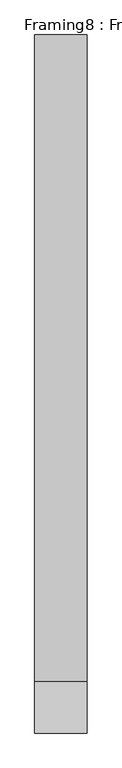
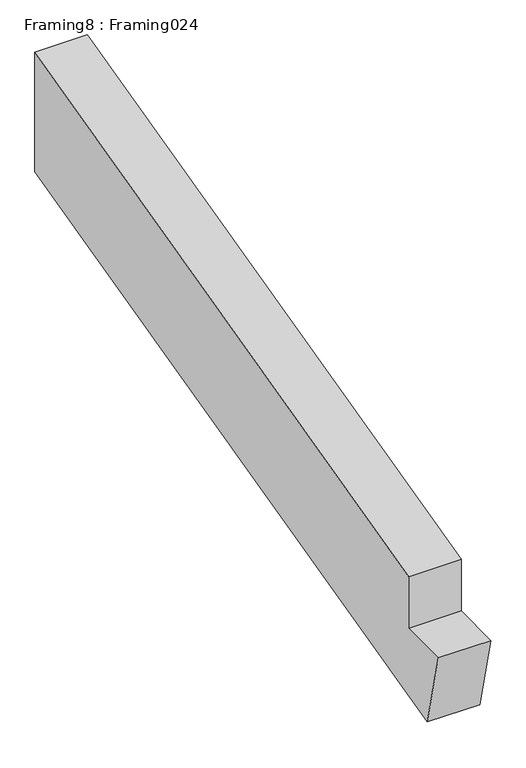
"""IFC4 building model written with IfcOpenShell, lengths in millimetres: proxy geometry, Framing8 : Framing024."""

import ifcopenshell
import ifcopenshell.guid

model = None  # the IFC model being written
_history = None  # IfcOwnerHistory: only IFC2X3 demands one
_inside = {}  # id of a spatial element -> (the spatial element, [elements in it])
_under = {}  # id of a project, library or spatial element -> (it, [spatial elements below it])
_declared = {}  # id of a project -> (the project, [libraries it declares])
_typed = {}  # id of a type object -> (the type object, [elements of that type])
_made_of = {}  # id of a material, layer set ... -> (it, [elements and type objects made of it])


def new_model(schema):
    """Start an empty IFC model of exactly this schema.

    Asked for "IFC4X3", IfcOpenShell would pick the latest addendum, in which some entities
    have other attributes; the version numbers below select the first issue.
    IFC2X3 requires an IfcOwnerHistory on every rooted entity: one is made here for all.
    """
    global model, _history
    if schema == "IFC4X3":
        model = ifcopenshell.file(schema_version=(4, 3, 0, 0))
    else:
        model = ifcopenshell.file(schema=schema)
    _inside.clear()
    _under.clear()
    _declared.clear()
    _typed.clear()
    _made_of.clear()
    _history = None
    if model.schema == "IFC2X3":
        org = make("IfcOrganization", Name="unknown")
        user = make(
            "IfcPersonAndOrganization",
            ThePerson=make("IfcPerson", FamilyName="unknown"),
            TheOrganization=org,
        )
        app = make(
            "IfcApplication",
            ApplicationDeveloper=org,
            Version="unknown",
            ApplicationFullName="unknown",
            ApplicationIdentifier="unknown",
        )
        _history = make(
            "IfcOwnerHistory",
            OwningUser=user,
            OwningApplication=app,
            ChangeAction="ADDED",
            CreationDate=0,
        )
    return model


def make(cls, **values):
    """One entity of the class cls with the attributes given. An attribute that is None is left unset."""
    return model.create_entity(
        cls, **{name: value for name, value in values.items() if value is not None}
    )


def rooted(cls, **values):
    """An entity with a GlobalId (a new one), such as an element, a storey or a relation."""
    return make(cls, GlobalId=ifcopenshell.guid.new(), OwnerHistory=_history, **values)


def si_unit(unit_type, name, prefix=None):
    """IfcSIUnit, for example si_unit("LENGTHUNIT", "METRE", prefix="MILLI")."""
    return make("IfcSIUnit", UnitType=unit_type, Prefix=prefix, Name=name)


def assignment(units):
    """IfcUnitAssignment: the units of a project."""
    return None if units is None else make("IfcUnitAssignment", Units=units)


def point(xyz):
    """IfcCartesianPoint."""
    return None if xyz is None else make("IfcCartesianPoint", Coordinates=xyz)


def direction(xyz):
    """IfcDirection."""
    return None if xyz is None else make("IfcDirection", DirectionRatios=xyz)


def frame(location, z_axis=None, x_axis=None):
    """IfcAxis2Placement3D, a coordinate frame: its origin and axes. An axis left out is left unset."""
    return make(
        "IfcAxis2Placement3D",
        Location=point(location),
        Axis=direction(z_axis),
        RefDirection=direction(x_axis),
    )


def origin():
    """The frame at (0, 0, 0) with its axes left unset."""
    return frame((0.0, 0.0, 0.0))


def place(relative_to, where):
    """IfcLocalPlacement: puts the frame where relative to a parent placement (None: the world)."""
    return make(
        "IfcLocalPlacement", PlacementRelTo=relative_to, RelativePlacement=where
    )


def context(
    kind, dimensions, precision=None, world=None, true_north=None, identifier=None
):
    """IfcGeometricRepresentationContext, for example the 3D "Model" context."""
    return make(
        "IfcGeometricRepresentationContext",
        ContextIdentifier=identifier,
        ContextType=kind,
        CoordinateSpaceDimension=dimensions,
        Precision=precision,
        WorldCoordinateSystem=world,
        TrueNorth=true_north,
    )


def project(units=None, contexts=None):
    """IfcProject with its units and contexts."""
    return rooted(
        "IfcProject",
        Name="project",
        RepresentationContexts=contexts,
        UnitsInContext=assignment(units),
    )


def spatial(cls, under=None, at=None, **own):
    """A site, building, storey or space (cls), placed at a placement, below another one or the project."""
    s = rooted(cls, ObjectPlacement=at, **own)
    if under is not None:
        _under.setdefault(under.id(), (under, []))[1].append(s)
    return s


def polyline(points):
    """IfcPolyline through the points."""
    return make("IfcPolyline", Points=[point(p) for p in points])


def outline(outer, holes=None, kind="AREA"):
    """IfcArbitraryClosedProfileDef: a profile drawn as a closed curve; with holes, ...WithVoids."""
    if holes is None:
        return make("IfcArbitraryClosedProfileDef", ProfileType=kind, OuterCurve=outer)
    return make(
        "IfcArbitraryProfileDefWithVoids",
        ProfileType=kind,
        OuterCurve=outer,
        InnerCurves=holes,
    )


def extrude(swept, where, along, depth):
    """IfcExtrudedAreaSolid: the profile swept, set in the frame where, extruded along a direction by depth."""
    return make(
        "IfcExtrudedAreaSolid",
        SweptArea=swept,
        Position=where,
        ExtrudedDirection=direction(along),
        Depth=depth,
    )


def shape(context_of_items, identifier, shape_type, items):
    """IfcShapeRepresentation: the items that make up one representation, for example the "Body"."""
    return make(
        "IfcShapeRepresentation",
        ContextOfItems=context_of_items,
        RepresentationIdentifier=identifier,
        RepresentationType=shape_type,
        Items=items,
    )


def source(mapping_origin, context_of_items, identifier, shape_type, items):
    """IfcRepresentationMap: a shape defined once, which mapped items show again and again."""
    return make(
        "IfcRepresentationMap",
        MappingOrigin=mapping_origin,
        MappedRepresentation=shape(context_of_items, identifier, shape_type, items),
    )


def transform(
    local_origin,
    x_axis=None,
    y_axis=None,
    z_axis=None,
    scale=None,
    scale2=None,
    scale3=None,
    uniform=True,
):
    """IfcCartesianTransformationOperator3D, or its non-uniform kind. x_axis, y_axis, z_axis: its Axis1, 2, 3."""
    if uniform:
        return make(
            "IfcCartesianTransformationOperator3D",
            Axis1=direction(x_axis),
            Axis2=direction(y_axis),
            LocalOrigin=point(local_origin),
            Scale=scale,
            Axis3=direction(z_axis),
        )
    return make(
        "IfcCartesianTransformationOperator3DnonUniform",
        Axis1=direction(x_axis),
        Axis2=direction(y_axis),
        LocalOrigin=point(local_origin),
        Scale=scale,
        Axis3=direction(z_axis),
        Scale2=scale2,
        Scale3=scale3,
    )


def mapped(mapping_source, mapping_target):
    """IfcMappedItem: shows the shape of a source again, moved by a transform."""
    return make(
        "IfcMappedItem", MappingSource=mapping_source, MappingTarget=mapping_target
    )


def made_of(thing, what):
    """Note that an element or type object is made of a material, layer set ...; save() writes the relation."""
    if what is not None:
        _made_of.setdefault(what.id(), (what, []))[1].append(thing)
    return thing


def element(
    cls,
    number,
    at=None,
    inside=None,
    cuts=None,
    type_object=None,
    material=None,
    context=None,
    identifier="Body",
    shape_type=None,
    held_by="IfcProductDefinitionShape",
    body=None,
    shapes=None,
    **own,
):
    """One element of the class cls, such as IfcWall. Its Tag is "e" and its number.

    at: its placement. inside: the storey or other place that contains it. cuts: it is an
    opening in that element (IfcRelVoidsElement). A single representation is given by context,
    identifier, shape_type and body (its items); several are given by shapes. held_by: the class
    of the entity that holds the representations. save() writes the other relations.
    """
    e = rooted(cls, Tag="e%d" % number, ObjectPlacement=at, **own)
    if body is not None:
        shapes = [shape(context, identifier, shape_type, body)]
    if shapes is not None:
        e.Representation = make(held_by, Representations=shapes)
    if inside is not None:
        _inside.setdefault(inside.id(), (inside, []))[1].append(e)
    if cuts is not None:
        rooted(
            "IfcRelVoidsElement", RelatingBuildingElement=cuts, RelatedOpeningElement=e
        )
    if type_object is not None:
        _typed.setdefault(type_object.id(), (type_object, []))[1].append(e)
    return made_of(e, material)


def aggregate(whole, parts):
    """IfcRelAggregates: a whole, such as a stair, and the parts it consists of."""
    return rooted("IfcRelAggregates", RelatingObject=whole, RelatedObjects=parts)


def save(model, path):
    """Write the relations noted so far, then the file.

    IfcRelAggregates (storeys below a building ...), IfcRelContainedInSpatialStructure (elements
    in a storey), IfcRelDefinesByType, IfcRelAssociatesMaterial and IfcRelDeclares: one each for
    every whole, place, type object, material and project.
    """
    for whole, parts in _under.values():
        aggregate(whole, parts)
    for where, things in _inside.values():
        rooted(
            "IfcRelContainedInSpatialStructure",
            RelatedElements=things,
            RelatingStructure=where,
        )
    for kind, things in _typed.values():
        rooted("IfcRelDefinesByType", RelatedObjects=things, RelatingType=kind)
    for what, things in _made_of.values():
        rooted("IfcRelAssociatesMaterial", RelatedObjects=things, RelatingMaterial=what)
    for by, libraries in _declared.values():
        rooted("IfcRelDeclares", RelatingContext=by, RelatedDefinitions=libraries)
    model.write(path)


def framing8_framing024_9f8700c4(model_context):
    return source(origin(), model_context, "Body", "SweptSolid", [
        extrude(outline(polyline([(-5374.9745897, 42642.0307603), (-5224.4076049, 42642.0307603), (-5224.4076049, 42800.8143799), (-3344.6566162, 43270.717426), (-3344.6566162, 42903.8818003), (-5318.455674, 42411.3663805), (-5374.9745897, 42642.0307603)])), frame((13534.9, 0.0, 0.0), z_axis=(1.0, 0.0, 0.0), x_axis=(0.0, 1.0, 0.0)), (0.0, 0.0, 1.0), 152.4),
    ])


if __name__ == "__main__":
    model = new_model("IFC4")
    model_context = context("Model", 3, world=origin())
    ifc_project = project(units=[si_unit("LENGTHUNIT", "METRE", prefix="MILLI")], contexts=[model_context])
    site = spatial("IfcSite", under=ifc_project)
    building = spatial("IfcBuilding", under=site)
    placement = place(None, origin())
    framing8_framing024_shape = framing8_framing024_9f8700c4(model_context)
    element("IfcBuildingElementProxy", 1, Name="Framing8 : Framing024", ObjectType="Framing8 : Framing024", at=placement, inside=building, context=model_context, shape_type="MappedRepresentation", body=[
        mapped(framing8_framing024_shape, transform((0.0, 0.0, 0.0), x_axis=(1.0, 0.0, 0.0), y_axis=(0.0, 1.0, 0.0), z_axis=(0.0, 0.0, 1.0))),
    ])
    save(model, "model.ifc")

# Revit data of these elements
# Type "Framing8 : Framing024"
#   NameOverride = "Framing024"
# Element 1 (IfcBuildingElementProxy, "Framing8 : Framing024")
#   Materials on its faces: "WOOD FRAMING (SEE STRUCT DWGS)"
# Materials
#   "WOOD FRAMING (SEE STRUCT DWGS)": class "Unassigned", colour RGB 224 188 168, transparency 0, Cost = 0
